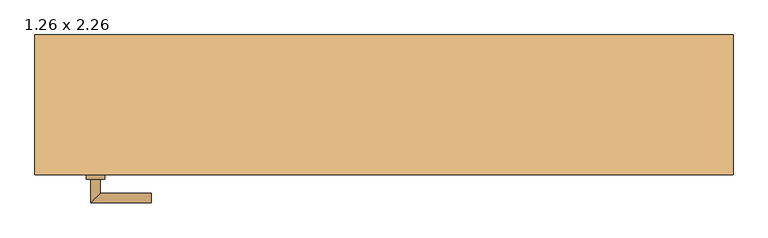
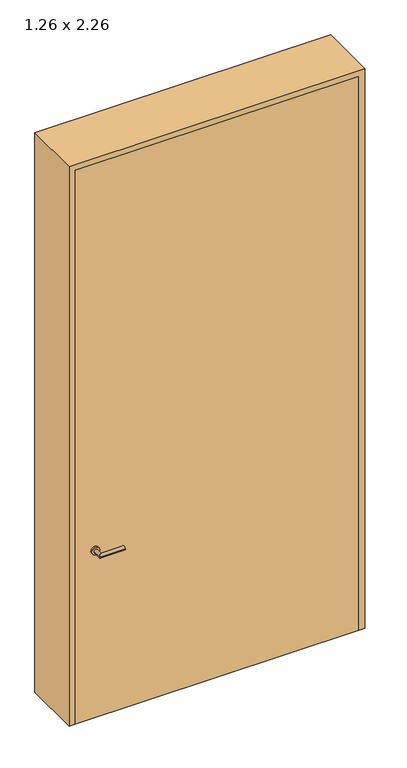
"""IFC4 building model written with IfcOpenShell, lengths in millimetres: door geometry, Drehflügel 1-flg - Blockzarge : 1.26 x 2.26."""

from ifc_helpers import new_model, si_unit, point, frame, frame_2d, origin, place, context, project, spatial, polyline, circle_curve, ellipse_curve, trimmed, segment, composite_curve, outline, extrude, source, transform, mapped, element, save
from ifc_brep_helpers import plane_surface, cylinder_surface, advanced_brep


def door_1_26_x_2_26_4041543f(model_context):
    return source(origin(), model_context, "Body", "SolidModel", [
        advanced_brep(
        [(-610.0, -129.4346141, 1000.0), (-630.0, -129.4346141, 1000.0), (-630.0, -79.4346141, 1000.0), (-610.0, -99.4346141, 1000.0), (-500.0, -99.4346141, 1000.0), (-500.0, -79.4346141, 1000.0)],
        [
            (0, 1, circle_curve(frame((-620.0, -129.4346141, 1000.0), z_axis=(0.0, -1.0, 0.0), x_axis=(-1.0, 0.0, 0.0)), 10.0)),
            (1, 0, circle_curve(frame((-620.0, -129.4346141, 1000.0), z_axis=(0.0, -1.0, 0.0), x_axis=(-1.0, 0.0, 0.0)), 10.0)),
            (1, 2),
            (2, 3, ellipse_curve(frame((-620.0, -89.4346141, 1000.0), z_axis=(-0.7071067811865686, -0.7071067811865265, 0.0), x_axis=(0.7071067811865264, -0.7071067811865687, 0.0)), 14.1421356, 10.0)),
            (3, 0),
            (3, 2, ellipse_curve(frame((-620.0, -89.4346141, 1000.0), z_axis=(-0.7071067811865686, -0.7071067811865265, 0.0), x_axis=(0.7071067811865264, -0.7071067811865687, 0.0)), 14.1421356, 10.0)),
            (4, 5, circle_curve(frame((-500.0, -89.4346141, 1000.0), z_axis=(1.0, 0.0, 0.0), x_axis=(0.0, 1.0, 0.0)), 10.0)),
            (5, 4, circle_curve(frame((-500.0, -89.4346141, 1000.0), z_axis=(1.0, 0.0, 0.0), x_axis=(0.0, 1.0, 0.0)), 10.0)),
            (2, 5),
            (4, 3),
        ],
        [
            plane_surface(frame((-620.0, -129.4346141, -287.7526403), z_axis=(0.0, -1.0, 0.0), x_axis=(0.0, 0.0, 1.0))),
            cylinder_surface(frame((-620.0, -129.4346141, 1000.0), z_axis=(0.0, -1.0, 0.0), x_axis=(-1.0, 0.0, 0.0)), 10.0),
            plane_surface(frame((-500.0, -89.4346141, -287.7526403), z_axis=(1.0, 0.0, 0.0), x_axis=(0.0, 0.0, 1.0))),
            cylinder_surface(frame((-620.0, -89.4346141, 1000.0), z_axis=(-1.0, 0.0, 0.0), x_axis=(0.0, 1.0, 0.0)), 10.0),
        ],
        [
            (0, [[1, 2]]),
            (1, [[3, 4, 5, -2]]),
            (1, [[-5, 6, -3, -1]]),
            (2, [[7, 8]]),
            (3, [[9, -7, 10, -4]]),
            (3, [[-10, -8, -9, -6]]),
        ],
    ),
        advanced_brep(
        [(-610.0, -174.4346141, 1000.0), (-630.0, -174.4346141, 1000.0), (-630.0, -224.4346141, 1000.0), (-610.0, -204.4346141, 1000.0), (-500.0, -204.4346141, 1000.0), (-500.0, -224.4346141, 1000.0)],
        [
            (0, 1, circle_curve(frame((-620.0, -174.4346141, 1000.0), z_axis=(0.0, 1.0, 0.0), x_axis=(-1.0, 0.0, 0.0)), 10.0)),
            (1, 0, circle_curve(frame((-620.0, -174.4346141, 1000.0), z_axis=(0.0, 1.0, 0.0), x_axis=(-1.0, 0.0, 0.0)), 10.0)),
            (1, 2),
            (2, 3, ellipse_curve(frame((-620.0, -214.4346141, 1000.0), z_axis=(-0.7071067811865486, 0.7071067811865464, 0.0), x_axis=(0.7071067811865464, 0.7071067811865488, 0.0)), 14.1421356, 10.0)),
            (3, 0),
            (3, 2, ellipse_curve(frame((-620.0, -214.4346141, 1000.0), z_axis=(-0.7071067811865486, 0.7071067811865464, 0.0), x_axis=(0.7071067811865464, 0.7071067811865488, 0.0)), 14.1421356, 10.0)),
            (4, 5, circle_curve(frame((-500.0, -214.4346141, 1000.0), z_axis=(1.0, 0.0, 0.0), x_axis=(0.0, -1.0, 0.0)), 10.0)),
            (5, 4, circle_curve(frame((-500.0, -214.4346141, 1000.0), z_axis=(1.0, 0.0, 0.0), x_axis=(0.0, -1.0, 0.0)), 10.0)),
            (2, 5),
            (4, 3),
        ],
        [
            plane_surface(frame((-620.0, -174.4346141, -287.7526403), z_axis=(0.0, 1.0, 0.0), x_axis=(0.0, 0.0, 1.0))),
            cylinder_surface(frame((-620.0, -174.4346141, 1000.0), z_axis=(0.0, 1.0, 0.0), x_axis=(-1.0, 0.0, 0.0)), 10.0),
            plane_surface(frame((-500.0, -214.4346141, -287.7526403), z_axis=(1.0, 0.0, 0.0), x_axis=(0.0, 0.0, 1.0))),
            cylinder_surface(frame((-620.0, -214.4346141, 1000.0), z_axis=(-1.0, 0.0, 0.0), x_axis=(0.0, -1.0, 0.0)), 10.0),
        ],
        [
            (0, [[1, 2]]),
            (1, [[3, 4, 5, -2]]),
            (1, [[-5, 6, -3, -1]]),
            (2, [[7, 8]]),
            (3, [[9, -7, 10, -4]]),
            (3, [[-10, -8, -9, -6]]),
        ],
    ),
        extrude(outline(composite_curve([segment(trimmed(circle_curve(frame_2d((1000.0, -620.0)), 20.0), [point((1000.0, -600.0))], [point((1000.0, -640.0))], False, "CARTESIAN"), True, "CONTINUOUS"), segment(trimmed(circle_curve(frame_2d((1000.0, -620.0)), 20.0), [point((1000.0, -640.0))], [point((1000.0, -600.0))], False, "CARTESIAN"), True, "CONTINUOUS")], self_intersect=False)), frame((0.0, -139.4346141, 0.0), z_axis=(0.0, 1.0, 0.0), x_axis=(0.0, 0.0, 1.0)), (0.0, 0.0, 1.0), 10.0),
        extrude(outline(composite_curve([segment(trimmed(circle_curve(frame_2d((1000.0, -620.0)), 20.0), [point((1000.0, -600.0))], [point((1000.0, -640.0))], False, "CARTESIAN"), True, "CONTINUOUS"), segment(trimmed(circle_curve(frame_2d((1000.0, -620.0)), 20.0), [point((1000.0, -640.0))], [point((1000.0, -600.0))], False, "CARTESIAN"), True, "CONTINUOUS")], self_intersect=False)), frame((0.0, -174.4346141, 0.0), z_axis=(0.0, 1.0, 0.0), x_axis=(0.0, 0.0, 1.0)), (0.0, 0.0, 1.0), 10.0),
        extrude(outline(polyline([(3100.0, 750.0), (3100.0, -750.0), (100.0, -750.0), (100.0, -720.0), (3070.0, -720.0), (3070.0, 720.0), (100.0, 720.0), (100.0, 750.0), (3100.0, 750.0)])), frame((0.0, -164.4346141, 0.0), z_axis=(0.0, 1.0, 0.0), x_axis=(0.0, 0.0, 1.0)), (0.0, 0.0, 1.0), 300.0),
        extrude(outline(polyline([(720.0, -164.4346141), (-720.0, -164.4346141), (-720.0, -139.4346141), (720.0, -139.4346141), (720.0, -164.4346141)])), frame((0.0, 0.0, 100.0), z_axis=(0.0, 0.0, 1.0), x_axis=(1.0, 0.0, 0.0)), (0.0, 0.0, 1.0), 2970.0),
    ])


if __name__ == "__main__":
    model = new_model("IFC4")
    model_context = context("Model", 3, world=origin())
    ifc_project = project(units=[si_unit("LENGTHUNIT", "METRE", prefix="MILLI")], contexts=[model_context])
    site = spatial("IfcSite", under=ifc_project)
    building = spatial("IfcBuilding", under=site)
    placement = place(None, origin())
    door_1_26_x_2_26_shape = door_1_26_x_2_26_4041543f(model_context)
    element("IfcDoor", 1, ObjectType="Drehflügel 1-flg - Blockzarge : 1.26 x 2.26", at=placement, inside=building, context=model_context, shape_type="MappedRepresentation", body=[
        mapped(door_1_26_x_2_26_shape, transform((0.0, 0.0, 0.0), x_axis=(1.0, 0.0, 0.0), y_axis=(0.0, 1.0, 0.0), z_axis=(0.0, 0.0, 1.0))),
    ])
    save(model, "model.ifc")

# Revit data of these elements
# Type "Drehflügel 1-flg - Blockzarge : 1.26 x 2.26"
#   Type Mark = "23"
#   Operation = "SingleSwingRight"
#   Keynote = "16.03"
#   Visual Light Transmittance = 0.9
#   Solar Heat Gain Coefficient = 0.86
#   Heat Transfer Coefficient (U) = 5.5617 W/(m²·K)
#   Rough Width = 1.500 m
#   Stärke Futter = 0.030 m
#   Rough Height [instance default] = 3.100 m
#   Höhe Türgriff = 0.900 m
#   Height = 3.000 m
#   Fußbodenaufbau [instance default] = 0.100 m
#   Width = 1.500 m
#   Sichtbarkeit Sturzlinien [instance default] = yes
#   Türgriff auswählen [instance default] = element 534090
#   Türgriff [instance default] = none
#   Türflügel [instance default] = none
#   Rahmen/Pfosten [instance default] = none
#   Construction Type Id = ""
#   Function = (empty or 0)
#   Wall Closure = (empty or 0)
#   Analytic Construction = (empty or 0)
# Element 1 (IfcDoor, "Drehflügel 1-flg - Blockzarge : 1.26 x 2.26")
#   Materials on its faces: "Metall - Chrom", "Holz - Birke"
# Materials
#   "Metall - Chrom": class "Metall", colour RGB 247 247 247, transparency 0, Cost = 0
#   "Holz - Birke": class "Holz", colour RGB 213 164 103, transparency 0, Cost = 0
